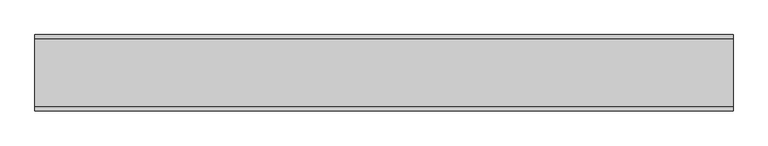
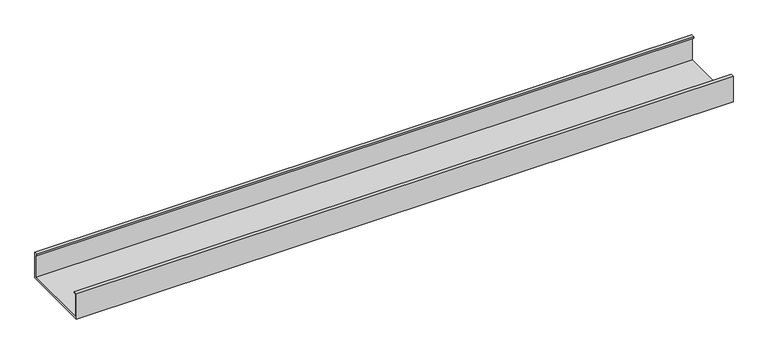
"""IFC4 building model written with IfcOpenShell, lengths in millimetres: proxy geometry, Generic Models 3:Generic Models 1:6:Generic Models 1:6 : Generic Models 3:Generic Models 1:300625:350611:Generic Models 1:6:Generic Models 1:6 : Generic Models 3:Generic Models 1:300625:350611 : Generic Models 3:Generic Models 1:6:Generic Models 1:6 : Generic Models 3:Generic Models 1:300625:350611:4 : Generic Models 3:Generic Models 1:6:Generic Models 1:6 : Generic Models 3:Generic Models 1:300625:350611:Generic Models 1:6:Generic Models 1:6 : Generic Models 3:Generic Models 1:300625:350611 : Generic Models 3:Generic Models 1:6:Generic Models 1:6 : Generic Models 3:Generic Models 1:300625:350611:301824."""

from ifc_helpers import new_model, si_unit, frame, origin, place, context, project, spatial, polyline, outline, extrude, source, transform, mapped, element, save


def generic_models_267f46cc(model_context):
    return source(origin(), model_context, "Body", "SweptSolid", [
        extrude(outline(polyline([(-536811.2913358, 0.0), (-536811.2913358, 95.25), (-536798.5913358, 95.25), (-536798.5913358, 90.4875), (-536806.5288358, 90.4875), (-536806.5288358, 4.7625), (-536562.0538841, 4.7625), (-536562.0538841, 90.4875), (-536569.9913841, 90.4875), (-536569.9913841, 95.25), (-536557.2913841, 95.25), (-536557.2913841, 0.0), (-536811.2913358, 0.0)])), frame((593853.2067753, 0.0, 0.0), z_axis=(1.0, 0.0, 0.0), x_axis=(0.0, 1.0, 0.0)), (0.0, 0.0, 1.0), 2323.2799489),
    ])


if __name__ == "__main__":
    model = new_model("IFC4")
    model_context = context("Model", 3, world=origin())
    ifc_project = project(units=[si_unit("LENGTHUNIT", "METRE", prefix="MILLI")], contexts=[model_context])
    site = spatial("IfcSite", under=ifc_project)
    building = spatial("IfcBuilding", under=site)
    placement = place(None, origin())
    generic_models_shape = generic_models_267f46cc(model_context)
    element("IfcBuildingElementProxy", 1, Name="Generic Models 3:Generic Models 1:6:Generic Models 1:6 : Generic Models 3:Generic Models 1:300625:350611:Generic Models 1:6:Generic Models 1:6 : Generic Models 3:Generic Models 1:300625:350611 : Generic Models 3:Generic Models 1:6:Generic Models 1:6 : Generic Models 3:Generic Models 1:300625:350611:4 : Generic Models 3:Generic Models 1:6:Generic Models 1:6 : Generic Models 3:Generic Models 1:300625:350611:Generic Models 1:6:Generic Models 1:6 : Generic Models 3:Generic Models 1:300625:350611 : Generic Models 3:Generic Models 1:6:Generic Models 1:6 : Generic Models 3:Generic Models 1:300625:350611:301824", ObjectType="Generic Models 3:Generic Models 1:6:Generic Models 1:6 : Generic Models 3:Generic Models 1:300625:350611:Generic Models 1:6:Generic Models 1:6 : Generic Models 3:Generic Models 1:300625:350611 : Generic Models 3:Generic Models 1:6:Generic Models 1:6 : Generic Models 3:Generic Models 1:300625:350611:4 : Generic Models 3:Generic Models 1:6:Generic Models 1:6 : Generic Models 3:Generic Models 1:300625:350611:Generic Models 1:6:Generic Models 1:6 : Generic Models 3:Generic Models 1:300625:350611 : Generic Models 3:Generic Models 1:6:Generic Models 1:6 : Generic Models 3:Generic Models 1:300625:350611:301824", at=placement, inside=building, context=model_context, shape_type="MappedRepresentation", body=[
        mapped(generic_models_shape, transform((0.0, 0.0, 0.0), x_axis=(1.0, 0.0, 0.0), y_axis=(0.0, 1.0, 0.0), z_axis=(0.0, 0.0, 1.0))),
    ])
    save(model, "model.ifc")

# Revit data of these elements
# Type "Generic Models 3:Generic Models 1:6:Generic Models 1:6 : Generic Models 3:Generic Models 1:300625:350611:Generic Models 1:6:Generic Models 1:6 : Generic Models 3:Generic Models 1:300625:350611 : Generic Models 3:Generic Models 1:6:Generic Models 1:6 : Generic Models 3:Generic Models 1:300625:350611:4 : Generic Models 3:Generic Models 1:6:Generic Models 1:6 : Generic Models 3:Generic Models 1:300625:350611:Generic Models 1:6:Generic Models 1:6 : Generic Models 3:Generic Models 1:300625:350611 : Generic Models 3:Generic Models 1:6:Generic Models 1:6 : Generic Models 3:Generic Models 1:300625:350611:301824"
#   NameOverride = "Generic Models 3:Generic Models 1:6:Generic Models 1:6 : Generic Models 3:Generic Models 1:300625:350611:Generic Models 1:6:Generic Models 1:6 : Generic Models 3:Generic Models 1:300625:350611 : Generic Models 3:Generic Models 1:6:Generic Models 1:6 : Generic Models 3:Generic Models 1:300625:350611:301824"
#   ObjectTypeOverride = "Generic Models 1:6:Generic Models 1:6 : Generic Models 3:Generic Models 1:300625:350611 : Generic Models 3:Generic Models 1:6:Generic Models 1:6 : Generic Models 3:Generic Models 1:300625:350611"
#   Reference = "Generic Models 1"
#   Tag = "301824"
